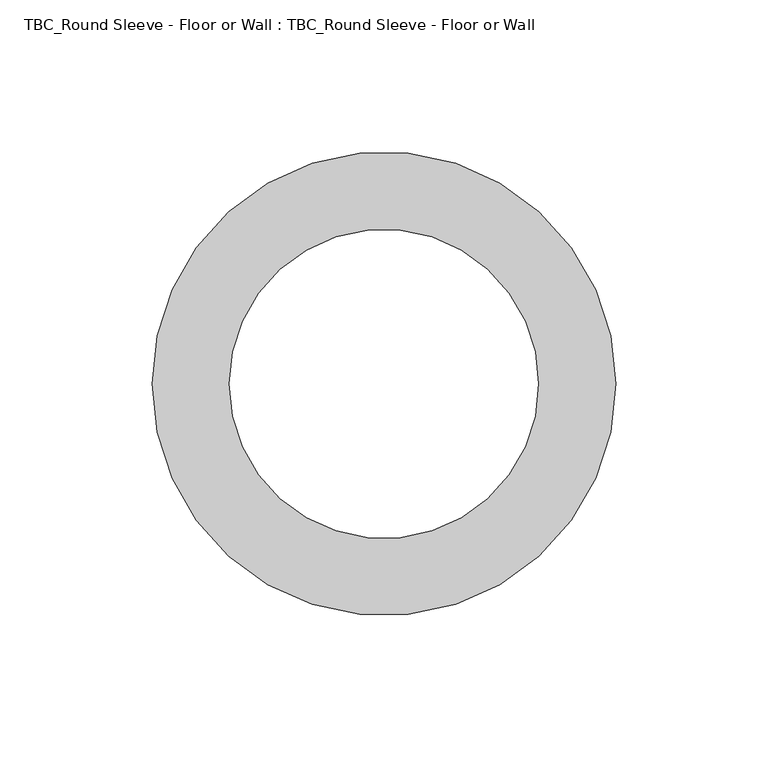
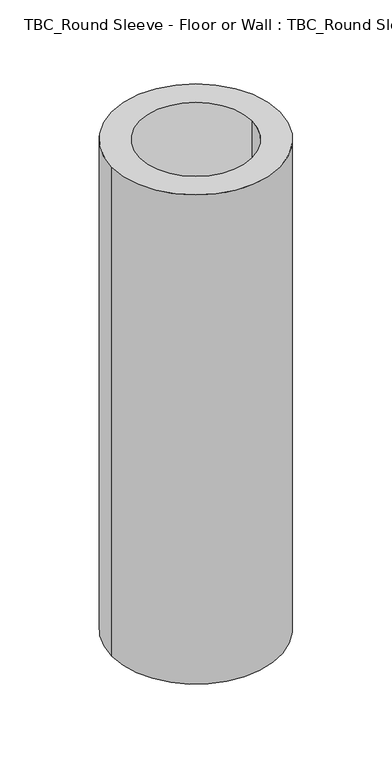
"""IFC4 building model written with IfcOpenShell, lengths in millimetres: proxy geometry, TBC_Round Sleeve - Floor or Wall : TBC_Round Sleeve - Floor or Wall."""

from ifc_helpers import new_model, si_unit, point, frame, origin, origin_2d, place, context, project, spatial, circle_curve, trimmed, segment, composite_curve, outline, extrude, source, transform, mapped, element, save


def tbc_round_sleeve_floor_or_wall_tbc_round_sleeve_floor_or_2b0a2645(model_context):
    return source(origin(), model_context, "Body", "SweptSolid", [
        extrude(outline(composite_curve([segment(trimmed(circle_curve(origin_2d(), 76.2), [point((-76.2, 0.0))], [point((76.2, 0.0))], False, "CARTESIAN"), True, "CONTINUOUS"), segment(trimmed(circle_curve(origin_2d(), 76.2), [point((76.2, 0.0))], [point((-76.2, 0.0))], False, "CARTESIAN"), True, "CONTINUOUS")], self_intersect=False), holes=[composite_curve([segment(trimmed(circle_curve(origin_2d(), 50.8), [point((-50.8, 0.0))], [point((50.8, 0.0))], True, "CARTESIAN"), True, "CONTINUOUS"), segment(trimmed(circle_curve(origin_2d(), 50.8), [point((50.8, 0.0))], [point((-50.8, 0.0))], True, "CARTESIAN"), True, "CONTINUOUS")], self_intersect=False)]), frame((0.0, 0.0, -469.9), z_axis=(0.0, 0.0, 1.0), x_axis=(1.0, 0.0, 0.0)), (0.0, 0.0, 1.0), 469.9),
    ])


if __name__ == "__main__":
    model = new_model("IFC4")
    model_context = context("Model", 3, world=origin())
    ifc_project = project(units=[si_unit("LENGTHUNIT", "METRE", prefix="MILLI")], contexts=[model_context])
    site = spatial("IfcSite", under=ifc_project)
    building = spatial("IfcBuilding", under=site)
    placement = place(None, origin())
    tbc_round_sleeve_floor_or_wall_tbc_round_sleeve_floor_or_shape = tbc_round_sleeve_floor_or_wall_tbc_round_sleeve_floor_or_2b0a2645(model_context)
    element("IfcBuildingElementProxy", 1, Name="TBC_Round Sleeve - Floor or Wall : TBC_Round Sleeve - Floor or Wall", ObjectType="TBC_Round Sleeve - Floor or Wall : TBC_Round Sleeve - Floor or Wall", at=placement, inside=building, context=model_context, shape_type="MappedRepresentation", body=[
        mapped(tbc_round_sleeve_floor_or_wall_tbc_round_sleeve_floor_or_shape, transform((0.0, 0.0, 0.0), x_axis=(1.0, 0.0, 0.0), y_axis=(0.0, 1.0, 0.0), z_axis=(0.0, 0.0, 1.0))),
    ])
    save(model, "model.ifc")

# Revit data of these elements
# Type "TBC_Round Sleeve - Floor or Wall : TBC_Round Sleeve - Floor or Wall"
#   Tag Dimension [instance default] = ""
#   MEP Type [instance default] = ""
#   MEP Element [instance default] = ""
#   MEP Category [instance default] = ""
#   Host Element Type [instance default] = ""
#   Host Element Id [instance default] = ""
#   Host Element Category [instance default] = ""
#   Control Line Y [instance default] = ""
#   Control Line X [instance default] = ""
#   Sleeve Radius [instance default] = 1' - 0"
#   Sleeve Edge [instance default] = 1' - 2"
#   Sleeve Depth [instance default] = 3' - 0"
#   Distance Y [instance default] = 0' - 0"
#   Distance X [instance default] = 0' - 0"
#   Default Elevation = 0
# Element 1 (IfcBuildingElementProxy, "TBC_Round Sleeve - Floor or Wall : TBC_Round Sleeve - Floor or Wall")
#   Tag Dimension = "6\""
#   MEP Type = "PLG-ST"
#   MEP Element = "820801"
#   MEP Category = "Pipe"
#   Host Element Type = "Roof System A"
#   Host Element Id = "1228029"
#   Host Element Category = "Roofs"
#   Sleeve Radius = 0' - 4"
#   Sleeve Edge = 0' - 6"
#   Sleeve Depth = 1' - 6 1/2"
